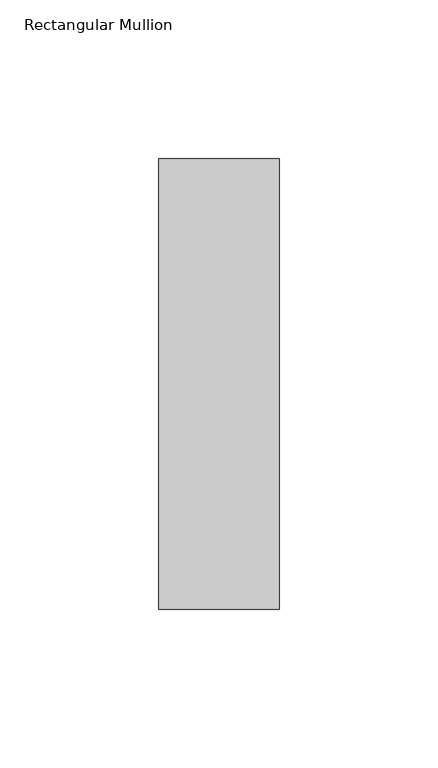
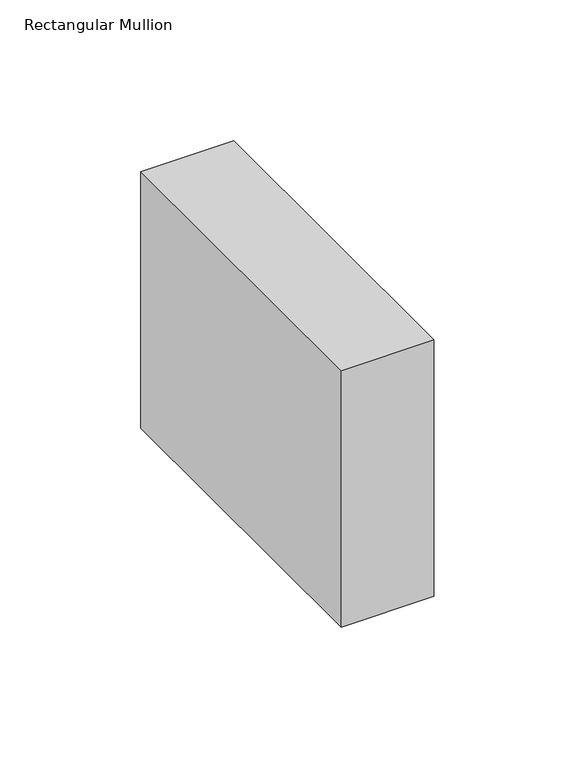
"""IFC4 building model written with IfcOpenShell, lengths in millimetres: member geometry, Rectangular Mullion : NLRS_21_CWM_hsb-regel 38x142_gen_rsf."""

import ifcopenshell
import ifcopenshell.guid

model = None  # the IFC model being written
_history = None  # IfcOwnerHistory: only IFC2X3 demands one
_inside = {}  # id of a spatial element -> (the spatial element, [elements in it])
_under = {}  # id of a project, library or spatial element -> (it, [spatial elements below it])
_declared = {}  # id of a project -> (the project, [libraries it declares])
_typed = {}  # id of a type object -> (the type object, [elements of that type])
_made_of = {}  # id of a material, layer set ... -> (it, [elements and type objects made of it])


def new_model(schema):
    """Start an empty IFC model of exactly this schema.

    Asked for "IFC4X3", IfcOpenShell would pick the latest addendum, in which some entities
    have other attributes; the version numbers below select the first issue.
    IFC2X3 requires an IfcOwnerHistory on every rooted entity: one is made here for all.
    """
    global model, _history
    if schema == "IFC4X3":
        model = ifcopenshell.file(schema_version=(4, 3, 0, 0))
    else:
        model = ifcopenshell.file(schema=schema)
    _inside.clear()
    _under.clear()
    _declared.clear()
    _typed.clear()
    _made_of.clear()
    _history = None
    if model.schema == "IFC2X3":
        org = make("IfcOrganization", Name="unknown")
        user = make(
            "IfcPersonAndOrganization",
            ThePerson=make("IfcPerson", FamilyName="unknown"),
            TheOrganization=org,
        )
        app = make(
            "IfcApplication",
            ApplicationDeveloper=org,
            Version="unknown",
            ApplicationFullName="unknown",
            ApplicationIdentifier="unknown",
        )
        _history = make(
            "IfcOwnerHistory",
            OwningUser=user,
            OwningApplication=app,
            ChangeAction="ADDED",
            CreationDate=0,
        )
    return model


def make(cls, **values):
    """One entity of the class cls with the attributes given. An attribute that is None is left unset."""
    return model.create_entity(
        cls, **{name: value for name, value in values.items() if value is not None}
    )


def rooted(cls, **values):
    """An entity with a GlobalId (a new one), such as an element, a storey or a relation."""
    return make(cls, GlobalId=ifcopenshell.guid.new(), OwnerHistory=_history, **values)


def si_unit(unit_type, name, prefix=None):
    """IfcSIUnit, for example si_unit("LENGTHUNIT", "METRE", prefix="MILLI")."""
    return make("IfcSIUnit", UnitType=unit_type, Prefix=prefix, Name=name)


def assignment(units):
    """IfcUnitAssignment: the units of a project."""
    return None if units is None else make("IfcUnitAssignment", Units=units)


def point(xyz):
    """IfcCartesianPoint."""
    return None if xyz is None else make("IfcCartesianPoint", Coordinates=xyz)


def direction(xyz):
    """IfcDirection."""
    return None if xyz is None else make("IfcDirection", DirectionRatios=xyz)


def frame(location, z_axis=None, x_axis=None):
    """IfcAxis2Placement3D, a coordinate frame: its origin and axes. An axis left out is left unset."""
    return make(
        "IfcAxis2Placement3D",
        Location=point(location),
        Axis=direction(z_axis),
        RefDirection=direction(x_axis),
    )


def origin():
    """The frame at (0, 0, 0) with its axes left unset."""
    return frame((0.0, 0.0, 0.0))


def place(relative_to, where):
    """IfcLocalPlacement: puts the frame where relative to a parent placement (None: the world)."""
    return make(
        "IfcLocalPlacement", PlacementRelTo=relative_to, RelativePlacement=where
    )


def context(
    kind, dimensions, precision=None, world=None, true_north=None, identifier=None
):
    """IfcGeometricRepresentationContext, for example the 3D "Model" context."""
    return make(
        "IfcGeometricRepresentationContext",
        ContextIdentifier=identifier,
        ContextType=kind,
        CoordinateSpaceDimension=dimensions,
        Precision=precision,
        WorldCoordinateSystem=world,
        TrueNorth=true_north,
    )


def project(units=None, contexts=None):
    """IfcProject with its units and contexts."""
    return rooted(
        "IfcProject",
        Name="project",
        RepresentationContexts=contexts,
        UnitsInContext=assignment(units),
    )


def spatial(cls, under=None, at=None, **own):
    """A site, building, storey or space (cls), placed at a placement, below another one or the project."""
    s = rooted(cls, ObjectPlacement=at, **own)
    if under is not None:
        _under.setdefault(under.id(), (under, []))[1].append(s)
    return s


def polyline(points):
    """IfcPolyline through the points."""
    return make("IfcPolyline", Points=[point(p) for p in points])


def outline(outer, holes=None, kind="AREA"):
    """IfcArbitraryClosedProfileDef: a profile drawn as a closed curve; with holes, ...WithVoids."""
    if holes is None:
        return make("IfcArbitraryClosedProfileDef", ProfileType=kind, OuterCurve=outer)
    return make(
        "IfcArbitraryProfileDefWithVoids",
        ProfileType=kind,
        OuterCurve=outer,
        InnerCurves=holes,
    )


def extrude(swept, where, along, depth):
    """IfcExtrudedAreaSolid: the profile swept, set in the frame where, extruded along a direction by depth."""
    return make(
        "IfcExtrudedAreaSolid",
        SweptArea=swept,
        Position=where,
        ExtrudedDirection=direction(along),
        Depth=depth,
    )


def shape(context_of_items, identifier, shape_type, items):
    """IfcShapeRepresentation: the items that make up one representation, for example the "Body"."""
    return make(
        "IfcShapeRepresentation",
        ContextOfItems=context_of_items,
        RepresentationIdentifier=identifier,
        RepresentationType=shape_type,
        Items=items,
    )


def source(mapping_origin, context_of_items, identifier, shape_type, items):
    """IfcRepresentationMap: a shape defined once, which mapped items show again and again."""
    return make(
        "IfcRepresentationMap",
        MappingOrigin=mapping_origin,
        MappedRepresentation=shape(context_of_items, identifier, shape_type, items),
    )


def transform(
    local_origin,
    x_axis=None,
    y_axis=None,
    z_axis=None,
    scale=None,
    scale2=None,
    scale3=None,
    uniform=True,
):
    """IfcCartesianTransformationOperator3D, or its non-uniform kind. x_axis, y_axis, z_axis: its Axis1, 2, 3."""
    if uniform:
        return make(
            "IfcCartesianTransformationOperator3D",
            Axis1=direction(x_axis),
            Axis2=direction(y_axis),
            LocalOrigin=point(local_origin),
            Scale=scale,
            Axis3=direction(z_axis),
        )
    return make(
        "IfcCartesianTransformationOperator3DnonUniform",
        Axis1=direction(x_axis),
        Axis2=direction(y_axis),
        LocalOrigin=point(local_origin),
        Scale=scale,
        Axis3=direction(z_axis),
        Scale2=scale2,
        Scale3=scale3,
    )


def mapped(mapping_source, mapping_target):
    """IfcMappedItem: shows the shape of a source again, moved by a transform."""
    return make(
        "IfcMappedItem", MappingSource=mapping_source, MappingTarget=mapping_target
    )


def made_of(thing, what):
    """Note that an element or type object is made of a material, layer set ...; save() writes the relation."""
    if what is not None:
        _made_of.setdefault(what.id(), (what, []))[1].append(thing)
    return thing


def element(
    cls,
    number,
    at=None,
    inside=None,
    cuts=None,
    type_object=None,
    material=None,
    context=None,
    identifier="Body",
    shape_type=None,
    held_by="IfcProductDefinitionShape",
    body=None,
    shapes=None,
    **own,
):
    """One element of the class cls, such as IfcWall. Its Tag is "e" and its number.

    at: its placement. inside: the storey or other place that contains it. cuts: it is an
    opening in that element (IfcRelVoidsElement). A single representation is given by context,
    identifier, shape_type and body (its items); several are given by shapes. held_by: the class
    of the entity that holds the representations. save() writes the other relations.
    """
    e = rooted(cls, Tag="e%d" % number, ObjectPlacement=at, **own)
    if body is not None:
        shapes = [shape(context, identifier, shape_type, body)]
    if shapes is not None:
        e.Representation = make(held_by, Representations=shapes)
    if inside is not None:
        _inside.setdefault(inside.id(), (inside, []))[1].append(e)
    if cuts is not None:
        rooted(
            "IfcRelVoidsElement", RelatingBuildingElement=cuts, RelatedOpeningElement=e
        )
    if type_object is not None:
        _typed.setdefault(type_object.id(), (type_object, []))[1].append(e)
    return made_of(e, material)


def aggregate(whole, parts):
    """IfcRelAggregates: a whole, such as a stair, and the parts it consists of."""
    return rooted("IfcRelAggregates", RelatingObject=whole, RelatedObjects=parts)


def save(model, path):
    """Write the relations noted so far, then the file.

    IfcRelAggregates (storeys below a building ...), IfcRelContainedInSpatialStructure (elements
    in a storey), IfcRelDefinesByType, IfcRelAssociatesMaterial and IfcRelDeclares: one each for
    every whole, place, type object, material and project.
    """
    for whole, parts in _under.values():
        aggregate(whole, parts)
    for where, things in _inside.values():
        rooted(
            "IfcRelContainedInSpatialStructure",
            RelatedElements=things,
            RelatingStructure=where,
        )
    for kind, things in _typed.values():
        rooted("IfcRelDefinesByType", RelatedObjects=things, RelatingType=kind)
    for what, things in _made_of.values():
        rooted("IfcRelAssociatesMaterial", RelatedObjects=things, RelatingMaterial=what)
    for by, libraries in _declared.values():
        rooted("IfcRelDeclares", RelatingContext=by, RelatedDefinitions=libraries)
    model.write(path)


def rectangular_mullion_3ccaa2f0(model_context):
    return source(origin(), model_context, "Body", "SweptSolid", [
        extrude(outline(polyline([(-38.0, -71.0), (-38.0, 71.0), (0.0, 71.0), (0.0, -71.0), (-38.0, -71.0)])), frame((0.0, 0.0, -111.0), z_axis=(0.0, 0.0, 1.0), x_axis=(1.0, 0.0, 0.0)), (0.0, 0.0, 1.0), 111.0),
    ])


if __name__ == "__main__":
    model = new_model("IFC4")
    model_context = context("Model", 3, world=origin())
    ifc_project = project(units=[si_unit("LENGTHUNIT", "METRE", prefix="MILLI")], contexts=[model_context])
    site = spatial("IfcSite", under=ifc_project)
    building = spatial("IfcBuilding", under=site)
    placement = place(None, origin())
    rectangular_mullion_shape = rectangular_mullion_3ccaa2f0(model_context)
    element("IfcMember", 1, ObjectType="Rectangular Mullion : NLRS_21_CWM_hsb-regel 38x142_gen_rsf", at=placement, inside=building, context=model_context, shape_type="MappedRepresentation", body=[
        mapped(rectangular_mullion_shape, transform((0.0, 0.0, 0.0), x_axis=(1.0, 0.0, 0.0), y_axis=(0.0, 1.0, 0.0), z_axis=(0.0, 0.0, 1.0))),
    ])
    save(model, "model.ifc")

# Revit data of these elements
# Type "Rectangular Mullion : NLRS_21_CWM_hsb-regel 38x142_gen_rsf"
#   Export Type to IFC As = "IfcWall"
#   Type IfcGUID = "07M7mRoiH1CR8m_RSKIwpF"
#   Assembly Code = "21.10"
#   built-in parameter 1007322 = 0.465879 (stored number, unit not read)
#   built-in parameter 1007321 = 0.062336 (stored number, unit not read)
#   built-in parameter 1007320 = 0.062336 (stored number, unit not read)
# Element 1 (IfcMember, "Rectangular Mullion : NLRS_21_CWM_hsb-regel 38x142_gen_rsf")
#   Materials on its faces: "NLRS_i2_hout naaldhout vuren_gen_rsf"
# Materials
#   "NLRS_i2_hout naaldhout vuren_gen_rsf": class "I - Hout", colour RGB 234 199 147, transparency 0, Keynote = "i2", Manufacturer = "Revit Standards Foundation", URL = "www.revitstandards.org", Description = "hout vuren", Cost = 0
